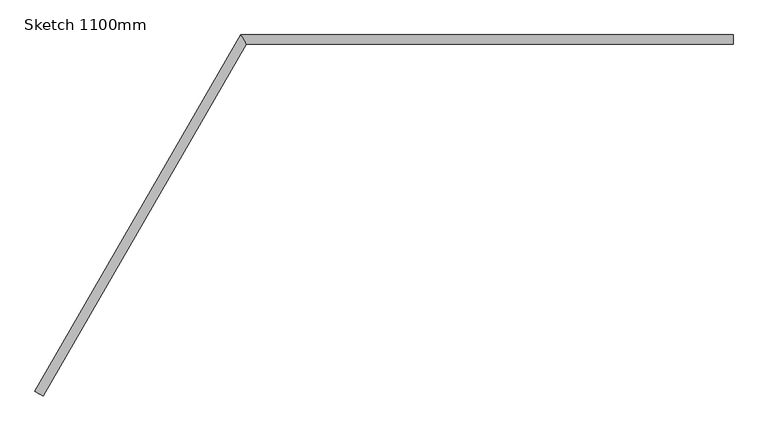
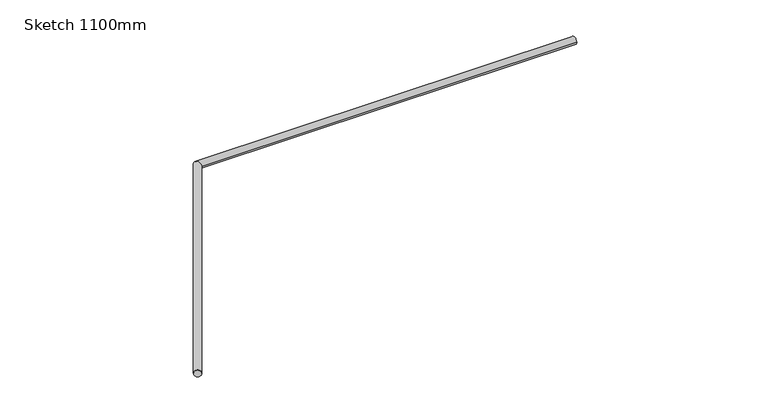
"""IFC4 building model written with IfcOpenShell, lengths in millimetres: railing geometry, Sketch 1100mm."""

from ifc_helpers import new_model, si_unit, frame, origin, place, context, project, spatial, circle_curve, ellipse_curve, source, transform, mapped, element, save
from ifc_brep_helpers import plane_surface, cylinder_surface, advanced_brep


def sketch_1100mm_c51240ad(model_context):
    return source(origin(), model_context, "Body", "AdvancedBrep", [
        advanced_brep(
        [(3000.0, 60.0, 4280.0), (2965.3589838, 80.0, 4280.0), (3842.931393, 1600.0, 4280.0), (3866.0254038, 1560.0, 4280.0), (5940.0, 1560.0, 4280.0), (5940.0, 1600.0, 4280.0)],
        [
            (0, 1, circle_curve(frame((2982.6794919, 70.0, 4280.0), z_axis=(-0.5000000000000013, -0.8660254037844379, 0.0), x_axis=(-0.8660254037844379, 0.5000000000000013, 0.0)), 20.0)),
            (1, 0, circle_curve(frame((2982.6794919, 70.0, 4280.0), z_axis=(-0.5000000000000013, -0.8660254037844379, 0.0), x_axis=(-0.8660254037844379, 0.5000000000000013, 0.0)), 20.0)),
            (1, 2),
            (2, 3, ellipse_curve(frame((3854.4783984, 1580.0, 4280.0), z_axis=(-0.8660254037844398, -0.49999999999999795, 0.0), x_axis=(0.4999999999999979, -0.8660254037844398, 0.0)), 23.0940108, 20.0)),
            (3, 0),
            (3, 2, ellipse_curve(frame((3854.4783984, 1580.0, 4280.0), z_axis=(-0.8660254037844398, -0.49999999999999795, 0.0), x_axis=(0.4999999999999979, -0.8660254037844398, 0.0)), 23.0940108, 20.0)),
            (4, 5, circle_curve(frame((5940.0, 1580.0, 4280.0), z_axis=(1.0, 0.0, 0.0), x_axis=(0.0, 1.0, 0.0)), 20.0)),
            (5, 4, circle_curve(frame((5940.0, 1580.0, 4280.0), z_axis=(1.0, 0.0, 0.0), x_axis=(0.0, 1.0, 0.0)), 20.0)),
            (2, 5),
            (4, 3),
        ],
        [
            plane_surface(frame((2982.6794919, 70.0, 4300.0), z_axis=(-0.5000000000000014, -0.8660254037844379, 0.0), x_axis=(0.8660254037844379, -0.5000000000000014, 0.0))),
            cylinder_surface(frame((2982.6794919, 70.0, 4280.0), z_axis=(-0.5000000000000013, -0.8660254037844379, 0.0), x_axis=(-0.8660254037844379, 0.5000000000000013, 0.0)), 20.0),
            plane_surface(frame((5940.0, 1580.0, 4300.0), z_axis=(1.0, 0.0, 0.0), x_axis=(0.0, 1.0, 0.0))),
            cylinder_surface(frame((3854.4783984, 1580.0, 4280.0), z_axis=(-1.0, 0.0, 0.0), x_axis=(0.0, 1.0, 0.0)), 20.0),
        ],
        [
            (0, [[1, 2]]),
            (1, [[-2, 3, 4, 5]]),
            (1, [[-1, -5, 6, -3]]),
            (2, [[7, 8]]),
            (3, [[-4, 9, -7, 10]]),
            (3, [[-6, -10, -8, -9]]),
        ],
    ),
    ])


if __name__ == "__main__":
    model = new_model("IFC4")
    model_context = context("Model", 3, world=origin())
    ifc_project = project(units=[si_unit("LENGTHUNIT", "METRE", prefix="MILLI")], contexts=[model_context])
    site = spatial("IfcSite", under=ifc_project)
    building = spatial("IfcBuilding", under=site)
    placement = place(None, origin())
    sketch_1100mm_shape = sketch_1100mm_c51240ad(model_context)
    element("IfcRailing", 1, ObjectType="Sketch 1100mm", at=placement, inside=building, context=model_context, shape_type="MappedRepresentation", body=[
        mapped(sketch_1100mm_shape, transform((0.0, 0.0, 0.0), x_axis=(1.0, 0.0, 0.0), y_axis=(0.0, 1.0, 0.0), z_axis=(0.0, 0.0, 1.0))),
    ])
    save(model, "model.ifc")

# Revit data of these elements
# Element 1 (IfcRailing, "Sketch 1100mm")
#   Materials on its faces: "Default Railings (Interior/Exterior)"
# Materials
#   "Default Railings (Interior/Exterior)": class "Generic", colour RGB 205 205 205, transparency 0, Description = "Udefineret gelænder materiale", Cost = 0
